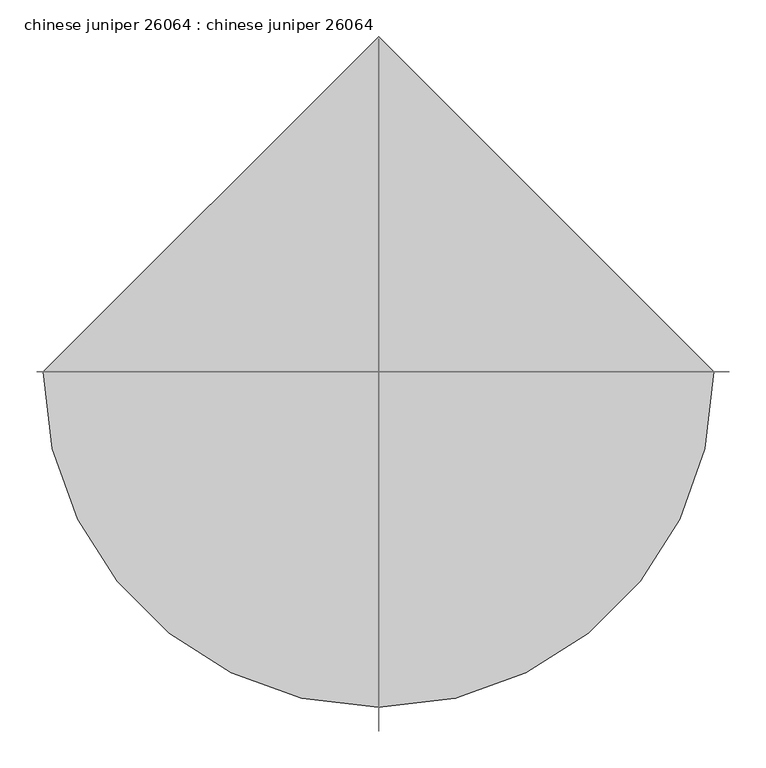
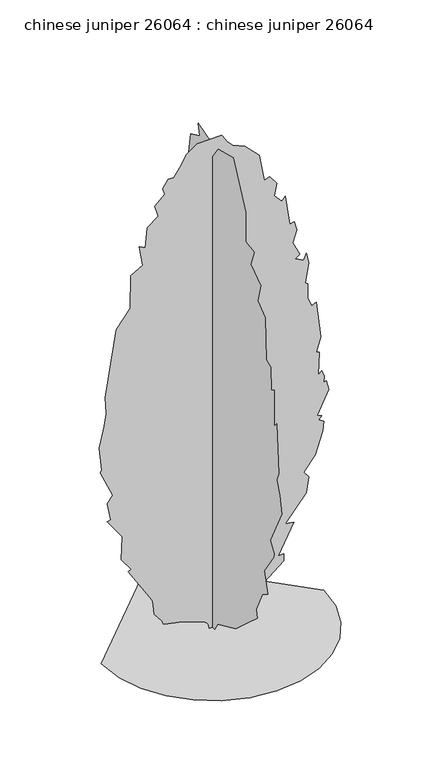
"""IFC4 building model written with IfcOpenShell, lengths in millimetres: proxy geometry, chinese juniper 26064 : chinese juniper 26064."""

import ifcopenshell
import ifcopenshell.guid

model = None  # the IFC model being written
_history = None  # IfcOwnerHistory: only IFC2X3 demands one
_inside = {}  # id of a spatial element -> (the spatial element, [elements in it])
_under = {}  # id of a project, library or spatial element -> (it, [spatial elements below it])
_declared = {}  # id of a project -> (the project, [libraries it declares])
_typed = {}  # id of a type object -> (the type object, [elements of that type])
_made_of = {}  # id of a material, layer set ... -> (it, [elements and type objects made of it])


def new_model(schema):
    """Start an empty IFC model of exactly this schema.

    Asked for "IFC4X3", IfcOpenShell would pick the latest addendum, in which some entities
    have other attributes; the version numbers below select the first issue.
    IFC2X3 requires an IfcOwnerHistory on every rooted entity: one is made here for all.
    """
    global model, _history
    if schema == "IFC4X3":
        model = ifcopenshell.file(schema_version=(4, 3, 0, 0))
    else:
        model = ifcopenshell.file(schema=schema)
    _inside.clear()
    _under.clear()
    _declared.clear()
    _typed.clear()
    _made_of.clear()
    _history = None
    if model.schema == "IFC2X3":
        org = make("IfcOrganization", Name="unknown")
        user = make(
            "IfcPersonAndOrganization",
            ThePerson=make("IfcPerson", FamilyName="unknown"),
            TheOrganization=org,
        )
        app = make(
            "IfcApplication",
            ApplicationDeveloper=org,
            Version="unknown",
            ApplicationFullName="unknown",
            ApplicationIdentifier="unknown",
        )
        _history = make(
            "IfcOwnerHistory",
            OwningUser=user,
            OwningApplication=app,
            ChangeAction="ADDED",
            CreationDate=0,
        )
    return model


def make(cls, **values):
    """One entity of the class cls with the attributes given. An attribute that is None is left unset."""
    return model.create_entity(
        cls, **{name: value for name, value in values.items() if value is not None}
    )


def rooted(cls, **values):
    """An entity with a GlobalId (a new one), such as an element, a storey or a relation."""
    return make(cls, GlobalId=ifcopenshell.guid.new(), OwnerHistory=_history, **values)


def si_unit(unit_type, name, prefix=None):
    """IfcSIUnit, for example si_unit("LENGTHUNIT", "METRE", prefix="MILLI")."""
    return make("IfcSIUnit", UnitType=unit_type, Prefix=prefix, Name=name)


def assignment(units):
    """IfcUnitAssignment: the units of a project."""
    return None if units is None else make("IfcUnitAssignment", Units=units)


def point(xyz):
    """IfcCartesianPoint."""
    return None if xyz is None else make("IfcCartesianPoint", Coordinates=xyz)


def direction(xyz):
    """IfcDirection."""
    return None if xyz is None else make("IfcDirection", DirectionRatios=xyz)


def frame(location, z_axis=None, x_axis=None):
    """IfcAxis2Placement3D, a coordinate frame: its origin and axes. An axis left out is left unset."""
    return make(
        "IfcAxis2Placement3D",
        Location=point(location),
        Axis=direction(z_axis),
        RefDirection=direction(x_axis),
    )


def origin():
    """The frame at (0, 0, 0) with its axes left unset."""
    return frame((0.0, 0.0, 0.0))


def place(relative_to, where):
    """IfcLocalPlacement: puts the frame where relative to a parent placement (None: the world)."""
    return make(
        "IfcLocalPlacement", PlacementRelTo=relative_to, RelativePlacement=where
    )


def context(
    kind, dimensions, precision=None, world=None, true_north=None, identifier=None
):
    """IfcGeometricRepresentationContext, for example the 3D "Model" context."""
    return make(
        "IfcGeometricRepresentationContext",
        ContextIdentifier=identifier,
        ContextType=kind,
        CoordinateSpaceDimension=dimensions,
        Precision=precision,
        WorldCoordinateSystem=world,
        TrueNorth=true_north,
    )


def project(units=None, contexts=None):
    """IfcProject with its units and contexts."""
    return rooted(
        "IfcProject",
        Name="project",
        RepresentationContexts=contexts,
        UnitsInContext=assignment(units),
    )


def spatial(cls, under=None, at=None, **own):
    """A site, building, storey or space (cls), placed at a placement, below another one or the project."""
    s = rooted(cls, ObjectPlacement=at, **own)
    if under is not None:
        _under.setdefault(under.id(), (under, []))[1].append(s)
    return s


def point_list(points):
    """IfcCartesianPointList2D or 3D."""
    cls = (
        "IfcCartesianPointList2D" if len(points[0]) == 2 else "IfcCartesianPointList3D"
    )
    return make(cls, CoordList=points)


def triangles(points, corners, closed=None, point_numbers=None):
    """IfcTriangulatedFaceSet: each triangle names its three corners, points numbered from 1."""
    return make(
        "IfcTriangulatedFaceSet",
        Coordinates=point_list(points),
        Closed=closed,
        CoordIndex=corners,
        PnIndex=point_numbers,
    )


def shape(context_of_items, identifier, shape_type, items):
    """IfcShapeRepresentation: the items that make up one representation, for example the "Body"."""
    return make(
        "IfcShapeRepresentation",
        ContextOfItems=context_of_items,
        RepresentationIdentifier=identifier,
        RepresentationType=shape_type,
        Items=items,
    )


def source(mapping_origin, context_of_items, identifier, shape_type, items):
    """IfcRepresentationMap: a shape defined once, which mapped items show again and again."""
    return make(
        "IfcRepresentationMap",
        MappingOrigin=mapping_origin,
        MappedRepresentation=shape(context_of_items, identifier, shape_type, items),
    )


def transform(
    local_origin,
    x_axis=None,
    y_axis=None,
    z_axis=None,
    scale=None,
    scale2=None,
    scale3=None,
    uniform=True,
):
    """IfcCartesianTransformationOperator3D, or its non-uniform kind. x_axis, y_axis, z_axis: its Axis1, 2, 3."""
    if uniform:
        return make(
            "IfcCartesianTransformationOperator3D",
            Axis1=direction(x_axis),
            Axis2=direction(y_axis),
            LocalOrigin=point(local_origin),
            Scale=scale,
            Axis3=direction(z_axis),
        )
    return make(
        "IfcCartesianTransformationOperator3DnonUniform",
        Axis1=direction(x_axis),
        Axis2=direction(y_axis),
        LocalOrigin=point(local_origin),
        Scale=scale,
        Axis3=direction(z_axis),
        Scale2=scale2,
        Scale3=scale3,
    )


def mapped(mapping_source, mapping_target):
    """IfcMappedItem: shows the shape of a source again, moved by a transform."""
    return make(
        "IfcMappedItem", MappingSource=mapping_source, MappingTarget=mapping_target
    )


def made_of(thing, what):
    """Note that an element or type object is made of a material, layer set ...; save() writes the relation."""
    if what is not None:
        _made_of.setdefault(what.id(), (what, []))[1].append(thing)
    return thing


def element(
    cls,
    number,
    at=None,
    inside=None,
    cuts=None,
    type_object=None,
    material=None,
    context=None,
    identifier="Body",
    shape_type=None,
    held_by="IfcProductDefinitionShape",
    body=None,
    shapes=None,
    **own,
):
    """One element of the class cls, such as IfcWall. Its Tag is "e" and its number.

    at: its placement. inside: the storey or other place that contains it. cuts: it is an
    opening in that element (IfcRelVoidsElement). A single representation is given by context,
    identifier, shape_type and body (its items); several are given by shapes. held_by: the class
    of the entity that holds the representations. save() writes the other relations.
    """
    e = rooted(cls, Tag="e%d" % number, ObjectPlacement=at, **own)
    if body is not None:
        shapes = [shape(context, identifier, shape_type, body)]
    if shapes is not None:
        e.Representation = make(held_by, Representations=shapes)
    if inside is not None:
        _inside.setdefault(inside.id(), (inside, []))[1].append(e)
    if cuts is not None:
        rooted(
            "IfcRelVoidsElement", RelatingBuildingElement=cuts, RelatedOpeningElement=e
        )
    if type_object is not None:
        _typed.setdefault(type_object.id(), (type_object, []))[1].append(e)
    return made_of(e, material)


def aggregate(whole, parts):
    """IfcRelAggregates: a whole, such as a stair, and the parts it consists of."""
    return rooted("IfcRelAggregates", RelatingObject=whole, RelatedObjects=parts)


def save(model, path):
    """Write the relations noted so far, then the file.

    IfcRelAggregates (storeys below a building ...), IfcRelContainedInSpatialStructure (elements
    in a storey), IfcRelDefinesByType, IfcRelAssociatesMaterial and IfcRelDeclares: one each for
    every whole, place, type object, material and project.
    """
    for whole, parts in _under.values():
        aggregate(whole, parts)
    for where, things in _inside.values():
        rooted(
            "IfcRelContainedInSpatialStructure",
            RelatedElements=things,
            RelatingStructure=where,
        )
    for kind, things in _typed.values():
        rooted("IfcRelDefinesByType", RelatedObjects=things, RelatingType=kind)
    for what, things in _made_of.values():
        rooted("IfcRelAssociatesMaterial", RelatedObjects=things, RelatingMaterial=what)
    for by, libraries in _declared.values():
        rooted("IfcRelDeclares", RelatingContext=by, RelatedDefinitions=libraries)
    model.write(path)


def chinese_juniper_26064_chinese_juniper_26064_15d4aa58(model_context):
    return source(origin(), model_context, "Body", "Tessellation", [
        triangles([(-14.7143181, 6e-07, 1.3e-06), (-18.2037808, -3e-07, 17.9396969), (-27.6190332, -6e-07, 30.3914521), (-123.7652017, 1.5e-06, 65.7757953), (-201.8727252, 3.9e-06, 82.3498608), (-209.3591505, 3.1e-06, 101.0656516), (-239.5230251, 2.1e-06, 139.6788561), (-246.7912588, -1e-06, 198.3880905), (-258.0216416, -1.9e-06, 220.8470939), (-347.8566379, -6.4e-06, 363.0865585), (-336.2335828, -7.4e-06, 370.071561), (-375.982174, -8.9e-06, 425.7942498), (-371.9537135, -1.5e-05, 524.6285151), (-433.95022, -1.74e-05, 610.1379032), (-418.976897, -1.83e-05, 613.8793173), (-433.3685695, -2.22e-05, 689.5207758), (-411.4889457, -2.49e-05, 718.6876728), (-463.8943952, -2.95e-05, 834.7279736), (-456.4089872, -3.02e-05, 842.2133451), (-467.6383527, -3.58e-05, 943.2777431), (-447.3233863, -4.19e-05, 1031.4541197), (-437.6916704, -4.53e-05, 1081.7767748), (-441.4356279, -4.94e-05, 1152.8969976), (-396.5181298, -6.81e-05, 1433.6338589), (-340.3712663, -7.5e-05, 1508.4981846), (-337.3359501, -8.35e-05, 1648.2265743), (-287.9657986, -8.74e-05, 1676.941246), (-302.9391579, -9.18e-05, 1763.0323574), (-277.3841226, -9.21e-05, 1748.371479), (-269.2510252, -9.76e-05, 1834.1525803), (-224.3317467, -0.0001015, 1867.8406403), (-239.3045792, -0.0001038, 1916.5022049), (-198.1295307, -0.0001078, 1953.9342224), (-205.6159378, -0.000109, 1980.1369835), (-183.1569344, -0.000112, 2013.8251888), (-160.697931, -0.000113, 2013.8251888), (-134.9295457, -0.0001161, 2047.2821583), (-109.0956393, -0.0001202, 2095.8470718), (-62.7453116, -0.0001241, 2127.2339642), (36.9177479, -0.0001285, 2128.801165), (60.1491719, -0.0001273, 2092.4307106), (82.6081753, -0.000127, 2069.9720524), (132.5409287, -0.0001279, 2048.8239246), (191.1599888, -0.0001268, 1987.6224277), (213.6190104, -0.0001209, 1871.5845978), (236.0780138, -0.0001223, 1879.070042), (263.4699646, -0.0001212, 1839.8828991), (254.7932958, -0.0001178, 1789.2351185), (284.7399962, -0.0001171, 1755.5469131), (299.7107939, -0.0001186, 1770.5202724), (318.4281289, -0.0001119, 1643.2505699), (337.1429023, -0.0001129, 1646.9946728), (347.3206967, -0.0001111, 1609.9130699), (330.592212, -0.0001074, 1559.0291119), (359.6016332, -0.000105, 1497.2687828), (339.9877141, -0.0001034, 1485.5084541), (374.5749925, -0.0001038, 1467.3220642), (385.8043579, -0.0001059, 1493.5248253), (397.0337597, -0.0001037, 1448.6072182), (382.0629438, -9.81e-05, 1366.2577389), (392.870678, -9.81e-05, 1357.3651131), (391.3695342, -9.44e-05, 1296.562429), (408.2631251, -9.28e-05, 1257.7053532), (426.980442, -9.41e-05, 1265.1907974), (445.6952153, -8.55e-05, 1107.9794632), (426.980442, -8.11e-05, 1048.0886421), (438.6365255, -8.14e-05, 1044.1287821), (434.4658499, -7.54e-05, 947.0217007), (449.4392092, -7.68e-05, 958.2511024), (460.6685746, -7.57e-05, 932.0483414), (456.9246171, -7.4e-05, 905.8481964), (468.1539825, -7.47e-05, 909.5896105), (479.383348, -7.27e-05, 868.4161062), (430.7218924, -6.48e-05, 771.0931223), (449.4392092, -6.52e-05, 763.6077507), (438.2098074, -6.38e-05, 748.6343914), (456.9246171, -6.39e-05, 737.4049896), (452.9875754, -6.13e-05, 697.0620306), (423.2364844, -5.44e-05, 602.6499518), (374.5749925, -4.87e-05, 542.7590944), (397.0337597, -4.81e-05, 516.5563697), (384.7578738, -4.37e-05, 451.166393), (299.7107939, -3.36e-05, 344.3717488), (333.4014519, -3.49e-05, 340.6277913), (269.7666369, -2.47e-05, 217.1038994), (292.2254042, -2.57e-05, 217.1038994), (292.2254042, -2.39e-05, 187.1584707), (127.5256825, -8.7e-06, 52.4044321), (127.5256825, -9.8e-06, 71.1202274), (15.2310573, -7e-07, 0.0), (1.1e-06, 13.7891713, 0.00013), (2.6e-06, 34.4811189, 14.2963339), (5.1e-06, 77.4229995, 29.9456808), (7.2e-06, 178.488651, 67.3772736), (1.16e-05, 230.8930831, 116.0384931), (1.08e-05, 208.4340797, 119.7817057), (1.93e-05, 288.5449239, 235.2565704), (2.08e-05, 264.5824875, 291.9663175), (2.39e-05, 331.9587347, 389.2892833), (2.56e-05, 324.4733268, 434.2067814), (3.03e-05, 373.1322753, 494.0976388), (3.42e-05, 389.4924685, 565.7309481), (3.3e-05, 380.6202267, 640.0820784), (3.96e-05, 440.5110841, 729.9170746), (4.37e-05, 444.2524981, 819.7546143), (4.59e-05, 422.6319428, 893.2725832), (4.85e-05, 455.4818636, 1010.6565519), (4.9e-05, 425.5377248, 1051.8300562), (5.26e-05, 388.1056346, 1171.611771), (5.33e-05, 414.3083593, 1253.9613956), (5.72e-05, 384.3616407, 1373.7430378), (5.87e-05, 346.932094, 1444.8632607), (6.04e-05, 328.2147772, 1594.5917667), (5.89e-05, 305.75601, 1583.362365), (6.48e-05, 305.75601, 1718.1148956), (6.33e-05, 260.8385118, 1729.3441521), (6.18e-05, 237.0752094, 1809.303661), (6.41e-05, 223.406676, 1875.3287006), (6.41e-05, 178.488651, 1920.2461624), (6.9e-05, 156.0296476, 2055.0011639), (6.35e-05, 92.3955867, 2084.9454117), (6.6e-05, 102.0598133, 2133.1292439), (6.08e-05, 11.3487565, 2104.2112415), (6.18e-05, 6.3027505, 2040.0278046), (5.86e-05, -38.6152347, 2103.6627285), (5.52e-05, -147.1670527, 2133.606831), (4.72e-05, -237.0033388, 1950.1902649), (4.17e-05, -237.0033388, 1822.9231785), (3.86e-05, -296.2055936, 1812.3847229), (3.68e-05, -270.691199, 1744.3175114), (3.55e-05, -342.8426634, 1695.0642677), (3.29e-05, -323.0966666, 1617.050425), (2.88e-05, -375.4995727, 1575.8744499), (2.47e-05, -382.9874877, 1396.2018414), (2.28e-05, -413.5488853, 1383.1639744), (1.83e-05, -416.6756204, 1283.9081142), (1.8e-05, -439.1343876, 1298.8788574), (1.51e-05, -439.1343876, 1141.6675959), (1.12e-05, -457.849161, 1164.1263994), (5.4e-06, -472.8225203, 954.5096884), (4.6e-06, -456.5690065, 918.855542), (1.2e-06, -480.3104716, 864.672076), (1.4e-06, -491.5398371, 789.8078957), (-2.2e-06, -412.9316628, 628.8526766), (-5.3e-06, -439.1343876, 583.9351785), (-1.8e-06, -436.9195155, 568.0778978), (-3.2e-06, -368.0141647, 467.8974212), (-8.1e-06, -394.2168895, 381.8038754), (-7.5e-06, -353.0408054, 355.6011506), (-5.6e-06, -311.8672648, 265.7661362), (-7.4e-06, -319.3526728, 232.0767318), (-7.1e-06, -244.4894916, 164.6997216), (-6.7e-06, -165.8828434, 93.5794897), (-3.6e-06, -34.8715179, 33.6886368), (-3e-07, -16.1562041, 0.0001282), (-458.1641127, 0.0, 0.0001492), (-446.0508259, -104.9808196, 0.0001424), (-411.5549664, -201.3891246, 0.0001352), (-357.4375574, -286.4621113, 0.0001277), (-286.4621113, -357.4375574, 0.0001204), (-201.3891246, -411.5549664, 0.0001134), (-104.9808196, -446.0508259, 0.0001072), (2.06e-05, -458.1641127, 0.0001019), (104.9808196, -446.0508259, 9.8e-05), (201.3891246, -411.5549664, 9.58e-05), (286.4621113, -357.4375574, 9.54e-05), (357.4375574, -286.4621113, 9.65e-05), (411.5549664, -201.3888702, 9.92e-05), (446.0508259, -104.9808196, 0.0001034), (458.1641127, 4.01e-05, 0.0001092), (-5.98e-05, 458.1641127, 0.0001565)], [[57, 58, 59], [27, 28, 29], [87, 88, 89], [49, 50, 51], [13, 14, 15], [83, 84, 85], [74, 75, 76], [63, 64, 65], [68, 69, 70], [71, 72, 73], [9, 10, 11], [85, 86, 87], [85, 87, 89], [51, 52, 53], [54, 55, 56], [90, 1, 2], [66, 67, 68], [45, 46, 47], [17, 18, 19], [68, 70, 71], [45, 47, 48], [31, 32, 33], [76, 77, 78], [89, 90, 2], [89, 2, 3], [57, 59, 60], [51, 53, 54], [25, 26, 27], [39, 40, 41], [56, 57, 60], [71, 73, 74], [34, 35, 36], [33, 34, 36], [4, 5, 6], [60, 61, 62], [80, 81, 82], [38, 39, 41], [37, 38, 41], [37, 41, 42], [29, 30, 31], [15, 16, 17], [36, 37, 42], [33, 36, 42], [31, 33, 42], [31, 42, 43], [31, 43, 44], [31, 44, 45], [29, 31, 45], [29, 45, 48], [27, 29, 48], [25, 27, 48], [25, 48, 49], [25, 49, 51], [25, 51, 54], [25, 54, 56], [25, 56, 60], [25, 60, 62], [24, 25, 62], [23, 24, 62], [22, 23, 62], [22, 62, 63], [22, 63, 65], [22, 65, 66], [22, 66, 68], [21, 22, 68], [20, 21, 68], [19, 20, 68], [17, 19, 68], [17, 68, 71], [17, 71, 74], [15, 17, 74], [13, 15, 74], [13, 74, 76], [13, 76, 78], [13, 78, 79], [13, 79, 80], [12, 13, 80], [11, 12, 80], [9, 11, 80], [9, 80, 82], [9, 82, 83], [9, 83, 85], [9, 85, 89], [9, 89, 3], [9, 3, 4], [8, 9, 4], [8, 4, 6], [7, 8, 6], [138, 139, 140], [94, 95, 96], [136, 137, 138], [121, 122, 123], [112, 113, 114], [128, 129, 130], [121, 123, 124], [125, 126, 127], [124, 125, 127], [114, 115, 116], [147, 148, 149], [130, 131, 132], [124, 127, 128], [134, 135, 136], [154, 155, 91], [154, 91, 92], [150, 151, 152], [96, 97, 98], [119, 120, 121], [119, 121, 124], [119, 124, 128], [118, 119, 128], [117, 118, 128], [116, 117, 128], [116, 128, 130], [114, 116, 130], [114, 130, 132], [112, 114, 132], [112, 132, 133], [112, 133, 134], [112, 134, 136], [111, 112, 136], [110, 111, 136], [109, 110, 136], [109, 136, 138], [109, 138, 140], [109, 140, 141], [108, 109, 141], [107, 108, 141], [106, 107, 141], [105, 106, 141], [104, 105, 141], [103, 104, 141], [103, 141, 142], [103, 142, 143], [103, 143, 144], [102, 103, 144], [101, 102, 144], [100, 101, 144], [100, 144, 145], [100, 145, 146], [100, 146, 147], [100, 147, 149], [100, 149, 150], [100, 150, 152], [100, 152, 153], [100, 153, 154], [99, 100, 154], [98, 99, 154], [96, 98, 154], [96, 154, 92], [96, 92, 93], [96, 93, 94], [170, 171, 156], [169, 170, 156], [169, 156, 157], [168, 169, 157], [168, 157, 158], [168, 158, 159], [167, 168, 159], [166, 167, 159], [166, 159, 160], [166, 160, 161], [166, 161, 162], [166, 162, 163], [166, 163, 164], [166, 164, 165]], closed=False),
    ])


if __name__ == "__main__":
    model = new_model("IFC4")
    model_context = context("Model", 3, world=origin())
    ifc_project = project(units=[si_unit("LENGTHUNIT", "METRE", prefix="MILLI")], contexts=[model_context])
    site = spatial("IfcSite", under=ifc_project)
    building = spatial("IfcBuilding", under=site)
    placement = place(None, origin())
    chinese_juniper_26064_chinese_juniper_26064_shape = chinese_juniper_26064_chinese_juniper_26064_15d4aa58(model_context)
    element("IfcBuildingElementProxy", 1, Name="chinese juniper 26064 : chinese juniper 26064", ObjectType="chinese juniper 26064 : chinese juniper 26064", at=placement, inside=building, context=model_context, shape_type="MappedRepresentation", body=[
        mapped(chinese_juniper_26064_chinese_juniper_26064_shape, transform((0.0, 0.0, 0.0), x_axis=(1.0, 0.0, 0.0), y_axis=(0.0, 1.0, 0.0), z_axis=(0.0, 0.0, 1.0))),
    ])
    save(model, "model.ifc")

# Revit data of these elements
# Type "chinese juniper 26064 : chinese juniper 26064"
#   built-in parameter 1005195 = "RPC-16-FUM3-UUQ0-UBF0-N000-ST1L-LVER-AU"
#   Height = 0
